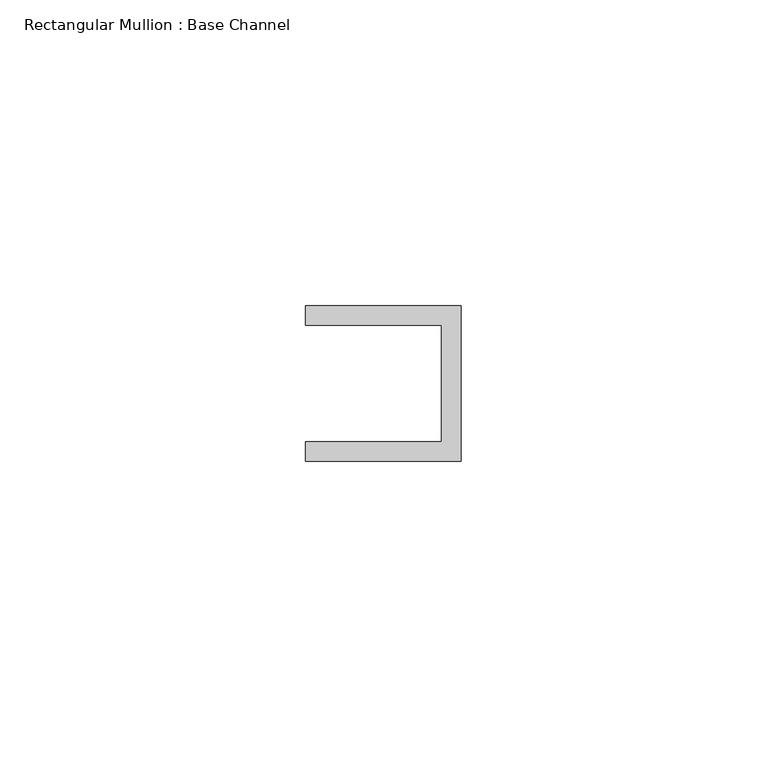
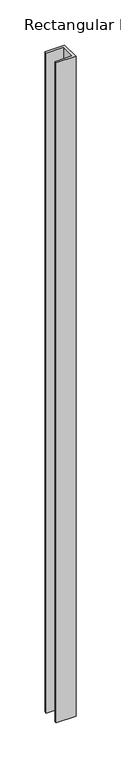
"""IFC4 building model written with IfcOpenShell, lengths in millimetres: member geometry, Rectangular Mullion : Base Channel."""

from ifc_helpers import new_model, si_unit, frame, origin, place, context, project, spatial, polyline, outline, extrude, source, transform, mapped, element, save


def rectangular_mullion_base_channel_39eeea65(model_context):
    return source(origin(), model_context, "Body", "SweptSolid", [
        extrude(outline(polyline([(0.0, -12.7), (-25.4, -12.7), (-25.4, -9.525), (-3.175, -9.525), (-3.175, 9.525), (-25.4, 9.525), (-25.4, 12.7), (0.0, 12.7), (0.0, -12.7)])), frame((0.0, 0.0, -894.3201523), z_axis=(0.0, 0.0, 1.0), x_axis=(1.0, 0.0, 0.0)), (0.0, 0.0, 1.0), 894.3201523),
    ])


if __name__ == "__main__":
    model = new_model("IFC4")
    model_context = context("Model", 3, world=origin())
    ifc_project = project(units=[si_unit("LENGTHUNIT", "METRE", prefix="MILLI")], contexts=[model_context])
    site = spatial("IfcSite", under=ifc_project)
    building = spatial("IfcBuilding", under=site)
    placement = place(None, origin())
    rectangular_mullion_base_channel_shape = rectangular_mullion_base_channel_39eeea65(model_context)
    element("IfcMember", 1, ObjectType="Rectangular Mullion : Base Channel", at=placement, inside=building, context=model_context, shape_type="MappedRepresentation", body=[
        mapped(rectangular_mullion_base_channel_shape, transform((0.0, 0.0, 0.0), x_axis=(1.0, 0.0, 0.0), y_axis=(0.0, 1.0, 0.0), z_axis=(0.0, 0.0, 1.0))),
    ])
    save(model, "model.ifc")

# Revit data of these elements
# Type "Rectangular Mullion : Base Channel"
#   built-in parameter 1007322 = 0.0833333 (stored number, unit not read)
#   built-in parameter 1007321 = 0.0416667 (stored number, unit not read)
#   built-in parameter 1007320 = -0.03125 (stored number, unit not read)
# Element 1 (IfcMember, "Rectangular Mullion : Base Channel")
#   Materials on its faces: "ALUM"
# Materials
#   "ALUM": class "Generic", colour RGB 157 157 157, transparency 0, Cost = 0
